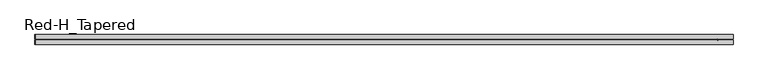
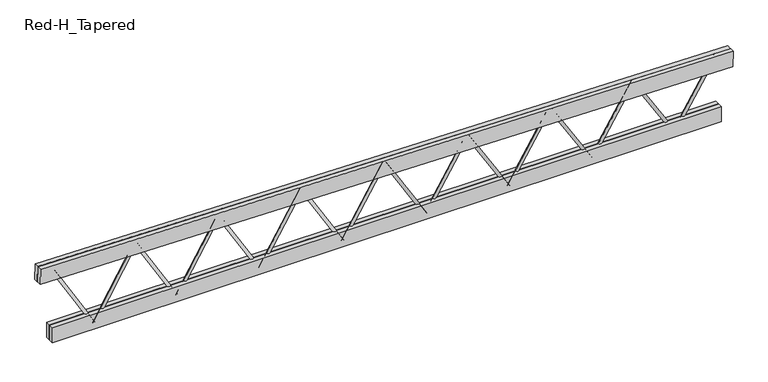
"""IFC4 building model written with IfcOpenShell, lengths in millimetres: beam geometry, Construction_Frames_RedBuilt_Openweb_Red-H_Tapered : Red-H_Tapered."""

from ifc_helpers import new_model, si_unit, point, frame, origin, origin_2d, place, context, project, spatial, polyline, circle_curve, trimmed, segment, composite_curve, outline, extrude, source, transform, mapped, element, save


def red_h_tapered_e310e839(model_context):
    return source(origin(), model_context, "Body", "SweptSolid", [
        extrude(outline(composite_curve([segment(trimmed(circle_curve(origin_2d(), 12.7), [point((0.0, 12.7))], [point((0.0, -12.7))], False, "CARTESIAN"), True, "CONTINUOUS"), segment(trimmed(circle_curve(origin_2d(), 12.7), [point((0.0, -12.7))], [point((0.0, 12.7))], False, "CARTESIAN"), True, "CONTINUOUS")], self_intersect=False)), frame((2516.6154336, 0.0, -367.0101562), z_axis=(0.5241067286958798, 0.0, 0.8516525916920017), x_axis=(0.0, -1.0, 0.0)), (0.0, 0.0, 1.0), 685.9604558),
        extrude(outline(composite_curve([segment(trimmed(circle_curve(origin_2d(), 12.7), [point((0.0, -12.7))], [point((0.0, 12.6999999))], False, "CARTESIAN"), True, "CONTINUOUS"), segment(trimmed(circle_curve(origin_2d(), 12.7), [point((0.0, 12.6999999))], [point((0.0, -12.7))], False, "CARTESIAN"), True, "CONTINUOUS")], self_intersect=False)), frame((2516.6154336, 0.0, -367.0101562), z_axis=(-0.5215353438102058, 0.0, 0.8532296790177722), x_axis=(0.0, -1.0, 0.0)), (0.0, 0.0, 1.0), 689.3425245),
        extrude(outline(composite_curve([segment(trimmed(circle_curve(origin_2d(), 12.7), [point((0.0, 12.7))], [point((0.0, -12.6999999))], False, "CARTESIAN"), True, "CONTINUOUS"), segment(trimmed(circle_curve(origin_2d(), 12.7), [point((0.0, -12.6999999))], [point((0.0, 12.7))], False, "CARTESIAN"), True, "CONTINUOUS")], self_intersect=False)), frame((1797.5824526, 0.0, -367.0101562), z_axis=(0.5215353438102048, 0.0, 0.8532296790177728), x_axis=(0.0, -1.0, 0.0)), (0.0, 0.0, 1.0), 689.3425245),
        extrude(outline(composite_curve([segment(trimmed(circle_curve(origin_2d(), 12.7), [point((0.0, -12.7))], [point((0.0, 12.7))], False, "CARTESIAN"), True, "CONTINUOUS"), segment(trimmed(circle_curve(origin_2d(), 12.7), [point((0.0, 12.7))], [point((0.0, -12.7))], False, "CARTESIAN"), True, "CONTINUOUS")], self_intersect=False)), frame((1797.5824526, 0.0, -367.0101562), z_axis=(-0.5189844139237986, 0.0, 0.8547837025260667), x_axis=(0.0, -1.0, 0.0)), (0.0, 0.0, 1.0), 692.7308044),
        extrude(outline(composite_curve([segment(trimmed(circle_curve(origin_2d(), 12.7), [point((0.0, 12.7000001))], [point((0.0, -12.7))], False, "CARTESIAN"), True, "CONTINUOUS"), segment(trimmed(circle_curve(origin_2d(), 12.7), [point((0.0, -12.7))], [point((0.0, 12.7000001))], False, "CARTESIAN"), True, "CONTINUOUS")], self_intersect=False)), frame((1078.5494715, 0.0, -367.0101562), z_axis=(0.5189844139237977, 0.0, 0.8547837025260674), x_axis=(0.0, -1.0, 0.0)), (0.0, 0.0, 1.0), 692.7308044),
        extrude(outline(composite_curve([segment(trimmed(circle_curve(origin_2d(), 12.7), [point((0.0, -12.7))], [point((0.0, 12.7))], False, "CARTESIAN"), True, "CONTINUOUS"), segment(trimmed(circle_curve(origin_2d(), 12.7), [point((0.0, 12.7))], [point((0.0, -12.7))], False, "CARTESIAN"), True, "CONTINUOUS")], self_intersect=False)), frame((1078.5494715, 0.0, -367.0101562), z_axis=(-0.5164537759218697, 0.0, 0.8563150689647142), x_axis=(0.0, -1.0, 0.0)), (0.0, 0.0, 1.0), 696.1252048),
        extrude(outline(composite_curve([segment(trimmed(circle_curve(origin_2d(), 12.7), [point((0.0, 12.7))], [point((0.0, -12.7))], False, "CARTESIAN"), True, "CONTINUOUS"), segment(trimmed(circle_curve(origin_2d(), 12.7), [point((0.0, -12.7))], [point((0.0, 12.7))], False, "CARTESIAN"), True, "CONTINUOUS")], self_intersect=False)), frame((359.5164905, 0.0, -367.0101562), z_axis=(0.5164537759218703, 0.0, 0.8563150689647139), x_axis=(0.0, -1.0, 0.0)), (0.0, 0.0, 1.0), 696.1252048),
        extrude(outline(composite_curve([segment(trimmed(circle_curve(origin_2d(), 12.7), [point((0.0, -12.7))], [point((0.0, 12.7))], False, "CARTESIAN"), True, "CONTINUOUS"), segment(trimmed(circle_curve(origin_2d(), 12.7), [point((0.0, 12.7))], [point((0.0, -12.7))], False, "CARTESIAN"), True, "CONTINUOUS")], self_intersect=False)), frame((359.5164905, 0.0, -367.0101562), z_axis=(-0.5139432662956573, 0.0, 0.8578241772236028), x_axis=(0.0, -1.0, 0.0)), (0.0, 0.0, 1.0), 699.5256366),
        extrude(outline(composite_curve([segment(trimmed(circle_curve(origin_2d(), 12.7), [point((0.0, -12.7))], [point((0.0, 12.7))], False, "CARTESIAN"), True, "CONTINUOUS"), segment(trimmed(circle_curve(origin_2d(), 12.7), [point((0.0, 12.7))], [point((0.0, -12.7))], False, "CARTESIAN"), True, "CONTINUOUS")], self_intersect=False)), frame((-359.5164905, 0.0, -367.0101562), z_axis=(0.5139432662956259, 0.0, 0.8578241772236216), x_axis=(0.0, -1.0, 0.0)), (0.0, 0.0, 1.0), 699.5256366),
        extrude(outline(composite_curve([segment(trimmed(circle_curve(origin_2d(), 12.7), [point((0.0, 12.7))], [point((0.0, -12.7))], False, "CARTESIAN"), True, "CONTINUOUS"), segment(trimmed(circle_curve(origin_2d(), 12.7), [point((0.0, -12.7))], [point((0.0, 12.7))], False, "CARTESIAN"), True, "CONTINUOUS")], self_intersect=False)), frame((-359.5164905, 0.0, -367.0101562), z_axis=(-0.5114527212428414, 0.0, 0.8593114184818519), x_axis=(0.0, -1.0, 0.0)), (0.0, 0.0, 1.0), 702.9320123),
        extrude(outline(composite_curve([segment(trimmed(circle_curve(origin_2d(), 12.7), [point((0.0, -12.7))], [point((0.0, 12.7))], False, "CARTESIAN"), True, "CONTINUOUS"), segment(trimmed(circle_curve(origin_2d(), 12.7), [point((0.0, 12.7))], [point((0.0, -12.7))], False, "CARTESIAN"), True, "CONTINUOUS")], self_intersect=False)), frame((-1078.5494715, 0.0, -367.0101562), z_axis=(0.5114527212428399, 0.0, 0.8593114184818528), x_axis=(0.0, -1.0, 0.0)), (0.0, 0.0, 1.0), 702.9320123),
        extrude(outline(composite_curve([segment(trimmed(circle_curve(origin_2d(), 12.7), [point((0.0, 12.7))], [point((0.0, -12.7000001))], False, "CARTESIAN"), True, "CONTINUOUS"), segment(trimmed(circle_curve(origin_2d(), 12.7), [point((0.0, -12.7000001))], [point((0.0, 12.7))], False, "CARTESIAN"), True, "CONTINUOUS")], self_intersect=False)), frame((-1078.5494715, 0.0, -367.0101562), z_axis=(-0.5089819767631923, 0.0, 0.8607771763529939), x_axis=(0.0, -1.0, 0.0)), (0.0, 0.0, 1.0), 706.3442458),
        extrude(outline(composite_curve([segment(trimmed(circle_curve(origin_2d(), 12.7), [point((0.0, -12.7))], [point((0.0, 12.7000001))], False, "CARTESIAN"), True, "CONTINUOUS"), segment(trimmed(circle_curve(origin_2d(), 12.7), [point((0.0, 12.7000001))], [point((0.0, -12.7))], False, "CARTESIAN"), True, "CONTINUOUS")], self_intersect=False)), frame((-1797.5824526, 0.0, -367.0101562), z_axis=(0.5089819767632053, 0.0, 0.8607771763529862), x_axis=(0.0, -1.0, 0.0)), (0.0, 0.0, 1.0), 706.3442458),
        extrude(outline(composite_curve([segment(trimmed(circle_curve(origin_2d(), 12.7), [point((0.0, 12.7))], [point((0.0, -12.7))], False, "CARTESIAN"), True, "CONTINUOUS"), segment(trimmed(circle_curve(origin_2d(), 12.7), [point((0.0, -12.7))], [point((0.0, 12.7))], False, "CARTESIAN"), True, "CONTINUOUS")], self_intersect=False)), frame((-1797.5824526, 0.0, -367.0101562), z_axis=(-0.5065308687490828, 0.0, 0.8622218270284622), x_axis=(0.0, -1.0, 0.0)), (0.0, 0.0, 1.0), 709.7622528),
        extrude(outline(composite_curve([segment(trimmed(circle_curve(origin_2d(), 12.7), [point((0.0, -12.7))], [point((0.0, 12.7))], False, "CARTESIAN"), True, "CONTINUOUS"), segment(trimmed(circle_curve(origin_2d(), 12.7), [point((0.0, 12.7))], [point((0.0, -12.7))], False, "CARTESIAN"), True, "CONTINUOUS")], self_intersect=False)), frame((-2516.6154336, 0.0, -367.0101562), z_axis=(0.5065308687490712, 0.0, 0.8622218270284691), x_axis=(0.0, -1.0, 0.0)), (0.0, 0.0, 1.0), 709.7622528),
        extrude(outline(composite_curve([segment(trimmed(circle_curve(origin_2d(), 12.7), [point((0.0, 12.7))], [point((0.0, -12.7))], False, "CARTESIAN"), True, "CONTINUOUS"), segment(trimmed(circle_curve(origin_2d(), 12.7), [point((0.0, -12.7))], [point((0.0, 12.7))], False, "CARTESIAN"), True, "CONTINUOUS")], self_intersect=False)), frame((-2516.6154336, 0.0, -367.0101562), z_axis=(-0.5040992330715786, 0.0, 0.863645739419032), x_axis=(0.0, -1.0, 0.0)), (0.0, 0.0, 1.0), 713.1859502),
        extrude(outline(polyline([(-2901.5319241, -41.275), (-2901.5319241, -3.175), (2901.5319241, -3.175), (2901.5319241, -41.275), (-2901.5319241, -41.275)])), frame((0.0, 0.0, -386.0601562), z_axis=(0.0, 0.0, 1.0), x_axis=(1.0, 0.0, 0.0)), (0.0, 0.0, 1.0), 139.7),
        extrude(outline(polyline([(-2901.5319241, 3.175), (-2901.5319241, 41.275), (2901.5319241, 41.275), (2901.5319241, 3.175), (-2901.5319241, 3.175)])), frame((0.0, 0.0, -386.0601562), z_axis=(0.0, 0.0, 1.0), x_axis=(1.0, 0.0, 0.0)), (0.0, 0.0, 1.0), 139.7),
        extrude(outline(polyline([(0.0, -38.1), (0.0, 0.0), (6007.123103, 0.0), (6007.123103, -38.1), (0.0, -38.1)])), frame((-3005.4947057, -3.175, 185.4598263), z_axis=(0.01691325419131241, 0.0, 0.9998569606862074), x_axis=(0.9998569606862074, 0.0, -0.01691325419131241)), (0.0, 0.0, 1.0), 139.7),
        extrude(outline(polyline([(0.0, -38.1), (0.0, 0.0), (6007.123103, 0.0), (6007.123103, -38.1), (0.0, -38.1)])), frame((-3005.4947057, 41.275, 185.4598263), z_axis=(0.01691325419131241, 0.0, 0.9998569606862074), x_axis=(0.9998569606862074, 0.0, -0.01691325419131241)), (0.0, 0.0, 1.0), 139.7),
    ])


if __name__ == "__main__":
    model = new_model("IFC4")
    model_context = context("Model", 3, world=origin())
    ifc_project = project(units=[si_unit("LENGTHUNIT", "METRE", prefix="MILLI")], contexts=[model_context])
    site = spatial("IfcSite", under=ifc_project)
    building = spatial("IfcBuilding", under=site)
    placement = place(None, origin())
    red_h_tapered_shape = red_h_tapered_e310e839(model_context)
    element("IfcBeam", 1, ObjectType="Construction_Frames_RedBuilt_Openweb_Red-H_Tapered : Red-H_Tapered", at=placement, inside=building, context=model_context, shape_type="MappedRepresentation", body=[
        mapped(red_h_tapered_shape, transform((0.0, 0.0, 0.0), x_axis=(1.0, 0.0, 0.0), y_axis=(0.0, 1.0, 0.0), z_axis=(0.0, 0.0, 1.0))),
    ])
    save(model, "model.ifc")

# Revit data of these elements
# Type "Construction_Frames_RedBuilt_Openweb_Red-H_Tapered : Red-H_Tapered"
#   Youtube clip = ""
#   Weight Net (Kg) = "0"
#   Webs = "Up to 2\" diameter tubular steel"
#   Uniformat II Description = ""
#   Uniformat II Code = ""
#   Uniclass 2015 Name = "Softwood trusses"
#   Uniclass 2015 Code = "Pr_20_85_90_81"
#   Uniclass 2.0 Description = "Structural Framing Systems"
#   Uniclass 2.0 Code = "SS-15-10-75"
#   Uniclass 1.4 Description = "Trusses"
#   Uniclass 1.4 Code = "L3523"
#   UNSPSC Code = "30103606"
#   Technical description = "http://www.redbuilt.com/reference/literature-and-other-resources"
#   Region South America = "None"
#   Region Oceania = "None"
#   Region North America = "US"
#   Region Middle East = "None"
#   Region Europe = "None"
#   Region Asia = "None"
#   Region Antarctica = "None"
#   Region Africa = "None"
#   QR code = "http://bimobject.com/redbuilt/product/redbuilt-0003"
#   Product url = "http://www.redbuilt.com/products/default.aspx?id=2"
#   Product group = "Wood Trusses"
#   Product family = "Construction"
#   Product data url = "https://bimobject.com/redbuilt/product/redbuilt-0003"
#   Product certification = ""
#   Product SKU = "redbuilt-0003"
#   Product Page URL = "http://www.redbuilt.com/commercial-systems/red-m-red-h-open-web-trusses"
#   Product Guid = "2c5793f2-6ffb-4665-b825-cf90c048e711"
#   Product Documentation Link = "http://www.redbuilt.com/documents/OW_Guide_2017_07_LowRes_wLinks.pdf"
#   OmniClass Description = "Wood Trusses"
#   OmniClass Code = "23-13 35 19 13 17"
#   NBS Reference Description = ""
#   NBS Reference Code = ""
#   Material secondary = "Steel"
#   Material main = "CHARRED WOOD"
#   Masterformat 2014 Description = "Metal-Web Wood Joists"
#   Masterformat 2014 Code = "06 17 36"
#   Manufacturer name = "RedBuilt"
#   Manufacturer country = "United States"
#   Installation instructions = "http://www.redbuilt.com/documents/Installation_Sheets_Open-Web.pdf"
#   IFC Classification = ""
#   EAN code = ""
#   Design country = "United States"
#   Product Information = "http://redbuilt.com/products/default.aspx?id=2"
#   Model = "Red-H-Tapered"
#   Manufacturer URL = "http://redbuilt.com/"
#   Manufacturer = "RedBuilt™"
#   Description = "Open Web Truss"
#   Date of publishing = "8/17/2010"
#   Contact us = "http://redbuilt.com/contact/"
#   Chords = "Double 1½\" x 5½\" MSR lumber"
#   COBIe Type Category = ""
#   Brand url = "http://www.redbuilt.com"
#   BIMobject main category code = "construction"
#   BIMobject main category = "Construction"
#   BIMobject category code = "construction-frames-trusses"
#   BIMobject category = "Frames & Trusses"
#   Web Radius = 0' - 0 1/2"
#   Web Layout Offset Start [instance default] = 0' - 5"
#   Web Layout Offset End [instance default] = 0' - 5"
#   Web Diameter = 0' - 1"
#   TotalLength [instance default] = 20' - 0"
#   Span Minimum = 4' - 0"
#   Span Maximum = 70' - 0"
#   Span Limit [instance default] = 20' - 0"
#   Nominal width = 0' - 0"
#   Nominal height = 0' - 0"
#   Inner Depth Top [instance default] = 0' - 2.76372"
#   Depth Start [instance default] = 6' - 0"
#   Top Chord Length [instance default] = 20' - 1.19701"
#   TC Extension Start Aux [instance default] = 0' - 0"
#   TC Extension End Aux [instance default] = 0' - 0"
#   T-B Chord Length Difference L [instance default] = 0' - 4"
#   T-B Chord Length Difference [instance default] = 0' - 4"
#   Height 2 [instance default] = 6' - 0"
#   Depth Minimum at Wall = 2' - 0"
#   Depth Maximum at Wall = 6' - 0"
#   Depth Lower End [instance default] = 2' - 0"
#   Depth Higher End [instance default] = 6' - 0"
#   Depth End [instance default] = 2' - 0"
#   Depth 2 [instance default] = 2' - 0"
#   Chord Width = 0' - 3 1/4"
#   Chord Thickness = 0' - 1 1/2"
#   Chord Depth = 0' - 5 1/2"
#   Offset Start [instance default] = 0' - 0"
#   TC Extension Start [instance default] = 0' - 0"
#   End Panel = 0' - 5"
#   Offset End [instance default] = 0' - 0"
#   TC Extension End [instance default] = 0' - 0"
#   Length [instance default] = 20' - 0"
#   Angle [instance default] = 5.71059°
#   Span Limit Warning [instance default] = no
#   Edition number = 1
#   Top Bearing Start [instance default] = yes
#   Top Bearing End [instance default] = yes
#   Bottom Bearing Start [instance default] = no
#   Bottom Bearing End [instance default] = no
#   8 Panels [instance default] = yes
#   16 Panels [instance default] = no
#   12 Panels [instance default] = no
#   Web Material = RedBuilt-Steel, Galvanized
#   Clip Material = RedBuilt-Steel, Galvanized
#   Chords Material = WOOD-OAKFIRE
#   URL = ""
#   Assembly Code = ""
# Element 1 (IfcBeam, "Construction_Frames_RedBuilt_Openweb_Red-H_Tapered : Red-H_Tapered")
#   TotalLength = 19' - 8.46708"
#   Span Limit = 19' - 8.46708"
#   Inner Depth Top = 0' - 2.75039"
#   Depth Start = 5' - 0"
#   Top Chord Length = 19' - 8.50091"
#   Height 2 = 5' - 0"
#   Depth Higher End = 5' - 0"
#   Depth 2 = 0' - 4"
#   Angle = 0.969104°
#   Materials on its faces: "RedBuilt-Steel, Galvanized", "WOOD-OAKFIRE"
# Materials
#   "RedBuilt-Steel, Galvanized": class "Metal", colour RGB 164 172 176, transparency 0, Manufacturer = "RedBuilt. LLC", Comments = "Openweb Metal Web", URL = "http://www.redbuilt.com/", Description = "Galvanized steel", Cost = 0
#   "WOOD-OAKFIRE": class "Wood", colour RGB 198 202 183, transparency 0, Description = "Generic wood", Cost = 0
